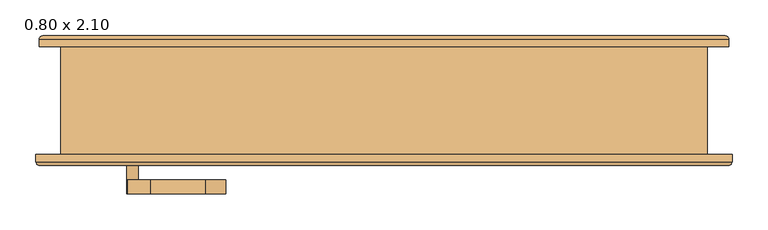
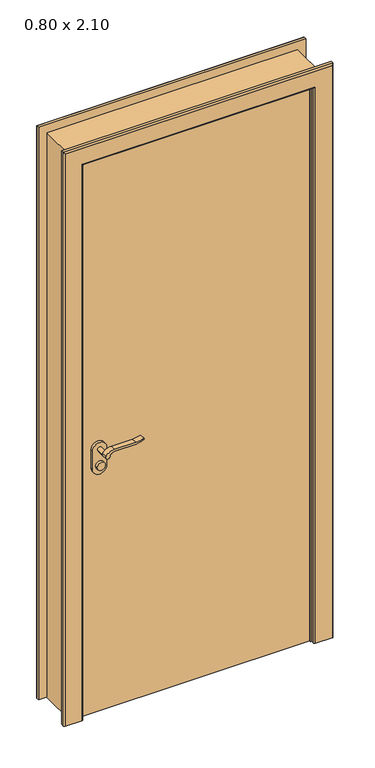
"""IFC4 building model written with IfcOpenShell, lengths in millimetres: door geometry, PORTA_DE_ABRIR_MADEIRA : 0.80 x 2.10."""

from ifc_helpers import new_model, si_unit, point, frame, frame_2d, origin, origin_with_axes, place, context, project, spatial, polyline, circle_curve, ellipse_curve, trimmed, segment, composite_curve, outline, extrude, faceted_brep, source, transform, mapped, element, save
from ifc_brep_helpers import plane_surface, cylinder_surface, advanced_brep


def door_0_80_x_2_10_69306b0e(model_context):
    return source(origin(), model_context, "Body", "SolidModel", [
        extrude(outline(composite_curve([segment(trimmed(circle_curve(frame_2d((940.0, -350.0)), 15.0), [point((940.0, -335.0))], [point((940.0, -365.0))], False, "CARTESIAN"), True, "CONTINUOUS"), segment(trimmed(circle_curve(frame_2d((940.0, -350.0)), 15.0), [point((940.0, -365.0))], [point((940.0, -335.0))], False, "CARTESIAN"), True, "CONTINUOUS")], self_intersect=False)), frame((0.0, -25.0, 0.0), z_axis=(0.0, 1.0, 0.0), x_axis=(0.0, 0.0, 1.0)), (0.0, 0.0, 1.0), 10.0),
        extrude(outline(composite_curve([segment(trimmed(circle_curve(frame_2d((940.0, -350.0)), 15.0), [point((940.0, -335.0))], [point((940.0, -365.0))], False, "CARTESIAN"), True, "CONTINUOUS"), segment(trimmed(circle_curve(frame_2d((940.0, -350.0)), 15.0), [point((940.0, -365.0))], [point((940.0, -335.0))], False, "CARTESIAN"), True, "CONTINUOUS")], self_intersect=False)), frame((0.0, -90.0, 0.0), z_axis=(0.0, 1.0, 0.0), x_axis=(0.0, 0.0, 1.0)), (0.0, 0.0, 1.0), 10.0),
        extrude(outline(composite_curve([segment(trimmed(circle_curve(frame_2d((1000.0, -350.0)), 8.0), [point((1004.6523287, -356.5081363))], [point((1000.0, -342.0))], False, "CARTESIAN"), True, "CONTINUOUS"), segment(trimmed(circle_curve(frame_2d((994.8738613, -324.6138099)), 18.1261387), [point((1000.0, -342.0))], [point((1013.0, -324.6138099))], True, "CARTESIAN"), True, "CONTINUOUS"), segment(polyline([(1013.0, -324.6138099), (1013.0, -248.3564091)]), True, "CONTINUOUS"), segment(trimmed(circle_curve(frame_2d((1072.2709207, -251.9396612)), 59.3791355), [point((1013.0, -248.3564091))], [point((1022.2135558, -220.0))], False, "CARTESIAN"), True, "CONTINUOUS"), segment(polyline([(1022.2135558, -220.0), (1025.0, -220.0)]), True, "CONTINUOUS"), segment(trimmed(circle_curve(frame_2d((1103.2850638, -248.4227909)), 83.2850902), [point((1025.0, -220.0))], [point((1020.0, -248.3564091))], True, "CARTESIAN"), True, "CONTINUOUS"), segment(polyline([(1020.0, -248.3564091), (1020.0, -324.6325667)]), True, "CONTINUOUS"), segment(trimmed(circle_curve(frame_2d((982.7555521, -326.3324871)), 37.2832219), [point((1020.0, -324.6325667))], [point((1004.6523287, -356.5081363))], False, "CARTESIAN"), True, "CONTINUOUS")], self_intersect=False)), frame((0.0, 5.0, 0.0), z_axis=(0.0, 1.0, 0.0), x_axis=(0.0, 0.0, 1.0)), (0.0, 0.0, 1.0), 20.0),
        extrude(outline(composite_curve([segment(trimmed(circle_curve(frame_2d((994.8738682, -324.6138122)), 18.1261318), [point((999.9999903, -342.0))], [point((1013.0, -324.6138122))], True, "CARTESIAN"), True, "CONTINUOUS"), segment(polyline([(1013.0, -324.6138122), (1013.0, -248.3564091)]), True, "CONTINUOUS"), segment(trimmed(circle_curve(frame_2d((1072.2709207, -251.9396612)), 59.3791355), [point((1013.0, -248.3564091))], [point((1022.2135558, -220.0))], False, "CARTESIAN"), True, "CONTINUOUS"), segment(polyline([(1022.2135558, -220.0), (1025.0, -220.0)]), True, "CONTINUOUS"), segment(trimmed(circle_curve(frame_2d((1103.2850638, -248.4227909)), 83.2850902), [point((1025.0, -220.0))], [point((1020.0, -248.3564091))], True, "CARTESIAN"), True, "CONTINUOUS"), segment(polyline([(1020.0, -248.3564091), (1020.0, -324.6325667)]), True, "CONTINUOUS"), segment(trimmed(circle_curve(frame_2d((982.7555521, -326.3324871)), 37.2832219), [point((1020.0, -324.6325667))], [point((1004.6523287, -356.5081363))], False, "CARTESIAN"), True, "CONTINUOUS"), segment(trimmed(circle_curve(frame_2d((1000.0, -350.0)), 8.0), [point((1004.6523287, -356.5081363))], [point((999.9999903, -342.0))], False, "CARTESIAN"), True, "CONTINUOUS")], self_intersect=False)), frame((0.0, -130.0, 0.0), z_axis=(0.0, 1.0, 0.0), x_axis=(0.0, 0.0, 1.0)), (0.0, 0.0, 1.0), 20.0),
        extrude(outline(composite_curve([segment(trimmed(circle_curve(frame_2d((1000.0, -350.0)), 8.0), [point((1000.0, -342.0))], [point((1000.0, -358.0))], False, "CARTESIAN"), True, "CONTINUOUS"), segment(trimmed(circle_curve(frame_2d((1000.0, -350.0)), 8.0), [point((1000.0, -358.0))], [point((1000.0, -342.0))], False, "CARTESIAN"), True, "CONTINUOUS")], self_intersect=False)), frame((0.0, -25.0, 0.0), z_axis=(0.0, 1.0, 0.0), x_axis=(0.0, 0.0, 1.0)), (0.0, 0.0, 1.0), 30.0),
        extrude(outline(composite_curve([segment(trimmed(circle_curve(frame_2d((1000.0, -350.0)), 8.0), [point((1000.0, -342.0))], [point((1000.0, -358.0))], False, "CARTESIAN"), True, "CONTINUOUS"), segment(trimmed(circle_curve(frame_2d((1000.0, -350.0)), 8.0), [point((1000.0, -358.0))], [point((1000.0, -342.0))], False, "CARTESIAN"), True, "CONTINUOUS")], self_intersect=False)), frame((0.0, -110.0, 0.0), z_axis=(0.0, 1.0, 0.0), x_axis=(0.0, 0.0, 1.0)), (0.0, 0.0, 1.0), 30.0),
        extrude(outline(composite_curve([segment(trimmed(circle_curve(frame_2d((930.0, -350.0)), 25.0), [point((930.0, -375.0))], [point((930.0, -325.0))], False, "CARTESIAN"), True, "CONTINUOUS"), segment(polyline([(930.0, -325.0), (1000.0, -325.0)]), True, "CONTINUOUS"), segment(trimmed(circle_curve(frame_2d((1000.0, -350.0)), 25.0), [point((1000.0, -325.0))], [point((1000.0, -375.0))], False, "CARTESIAN"), True, "CONTINUOUS"), segment(polyline([(1000.0, -375.0), (930.0, -375.0)]), True, "CONTINUOUS")], self_intersect=False)), frame((0.0, -35.0, 0.0), z_axis=(0.0, 1.0, 0.0), x_axis=(0.0, 0.0, 1.0)), (0.0, 0.0, 1.0), 10.0),
        extrude(outline(composite_curve([segment(trimmed(circle_curve(frame_2d((930.0, -350.0)), 25.0), [point((930.0, -375.0))], [point((930.0, -325.0))], False, "CARTESIAN"), True, "CONTINUOUS"), segment(polyline([(930.0, -325.0), (1000.0, -325.0)]), True, "CONTINUOUS"), segment(trimmed(circle_curve(frame_2d((1000.0, -350.0)), 25.0), [point((1000.0, -325.0))], [point((1000.0, -375.0))], False, "CARTESIAN"), True, "CONTINUOUS"), segment(polyline([(1000.0, -375.0), (930.0, -375.0)]), True, "CONTINUOUS")], self_intersect=False)), frame((0.0, -80.0, 0.0), z_axis=(0.0, 1.0, 0.0), x_axis=(0.0, 0.0, 1.0)), (0.0, 0.0, 1.0), 10.0),
        faceted_brep([(-410.0, -35.0, 0.0), (-410.0, -75.0, 0.0), (-450.0, -75.0, 0.0), (-450.0, 75.0, 0.0), (-400.0, 75.0, 0.0), (-400.0, -35.0, 0.0), (-410.0, -35.0, 2100.0), (-410.0, -75.0, 2100.0), (410.0, -75.0, 2100.0), (410.0, -75.0, 0.0), (450.0, -75.0, 0.0), (450.0, -75.0, 2140.0), (-450.0, -75.0, 2140.0), (-450.0, 75.0, 2140.0), (450.0, 75.0, 2140.0), (450.0, 75.0, 0.0), (400.0, 75.0, 0.0), (400.0, 75.0, 2090.0), (-400.0, 75.0, 2090.0), (-400.0, -35.0, 2090.0), (400.0, -35.0, 2090.0), (400.0, -35.0, 0.0), (410.0, -35.0, 0.0), (410.0, -35.0, 2100.0)], [[[0, 1, 2, 3, 4, 5]], [[1, 0, 6, 7]], [[2, 1, 7, 8, 9, 10, 11, 12]], [[3, 2, 12, 13]], [[4, 3, 13, 14, 15, 16, 17, 18]], [[5, 4, 18, 19]], [[0, 5, 19, 20, 21, 22, 23, 6]], [[20, 17, 16, 21]], [[22, 21, 16, 15, 10, 9]], [[8, 23, 22, 9]], [[14, 11, 10, 15]], [[13, 12, 11, 14]], [[19, 18, 17, 20]], [[7, 6, 23, 8]]]),
        advanced_brep(
        [(-480.0, 75.3, 0.0), (-480.0, 85.3, 0.0), (-475.0, 90.3, 0.0), (-415.0, 90.3, 0.0), (-410.0, 85.3, 0.0), (-410.0, 75.3, 0.0), (-480.0, 75.3, 2170.0), (-480.0, 85.3, 2170.0), (-475.0, 90.3, 2165.0), (475.0, 90.3, 2165.0), (475.0, 90.3, 0.0), (415.0, 90.3, 0.0), (415.0, 90.3, 2105.0), (-415.0, 90.3, 2105.0), (-410.0, 85.3, 2100.0), (-410.0, 75.3, 2100.0), (410.0, 75.3, 2100.0), (410.0, 75.3, 0.0), (480.0, 75.3, 0.0), (480.0, 75.3, 2170.0), (410.0, 85.3, 0.0), (480.0, 85.3, 0.0), (410.0, 85.3, 2100.0), (480.0, 85.3, 2170.0)],
        [
            (0, 1),
            (1, 2, circle_curve(frame((-475.0, 85.3, 0.0), z_axis=(0.0, 0.0, -1.0), x_axis=(-1.0, 0.0, 0.0)), 5.0)),
            (2, 3),
            (3, 4, circle_curve(frame((-415.0, 85.3, 0.0), z_axis=(0.0, 0.0, -1.0), x_axis=(-1.0, 0.0, 0.0)), 5.0)),
            (4, 5),
            (5, 0),
            (0, 6),
            (6, 7),
            (7, 1),
            (7, 8, ellipse_curve(frame((-475.0, 85.3, 2165.0), z_axis=(-0.7071067811865475, 0.0, -0.7071067811865475), x_axis=(0.7071067811865474, 0.0, -0.7071067811865476)), 7.0710678, 5.0)),
            (8, 2),
            (8, 9),
            (9, 10),
            (10, 11),
            (11, 12),
            (12, 13),
            (13, 3),
            (13, 14, ellipse_curve(frame((-415.0, 85.3, 2105.0), z_axis=(-0.7071067811865475, 0.0, -0.7071067811865475), x_axis=(0.7071067811865474, 0.0, -0.7071067811865476)), 7.0710678, 5.0)),
            (14, 4),
            (14, 15),
            (15, 5),
            (15, 16),
            (16, 17),
            (17, 18),
            (18, 19),
            (19, 6),
            (17, 20),
            (20, 11, circle_curve(frame((415.0, 85.3, 0.0), z_axis=(0.0, 0.0, -1.0), x_axis=(1.0, 0.0, 0.0)), 5.0)),
            (10, 21, circle_curve(frame((475.0, 85.3, 0.0), z_axis=(0.0, 0.0, -1.0), x_axis=(1.0, 0.0, 0.0)), 5.0)),
            (21, 18),
            (16, 22),
            (22, 20),
            (22, 12, ellipse_curve(frame((415.0, 85.3, 2105.0), z_axis=(0.7071067811865475, 0.0, -0.7071067811865475), x_axis=(0.7071067811865474, 0.0, 0.7071067811865476)), 7.0710678, 5.0)),
            (9, 23, ellipse_curve(frame((475.0, 85.3, 2165.0), z_axis=(0.7071067811865475, 0.0, -0.7071067811865475), x_axis=(0.7071067811865474, 0.0, 0.7071067811865476)), 7.0710678, 5.0)),
            (23, 21),
            (23, 19),
            (23, 7),
            (14, 22),
        ],
        [
            plane_surface(frame((-450.0, -75.0, 0.0), z_axis=(0.0, 0.0, -1.0), x_axis=(0.0, -1.0, 0.0))),
            plane_surface(frame((-480.0, 75.3, 0.0), z_axis=(-1.0, 0.0, 0.0), x_axis=(0.0, 0.0, 1.0))),
            cylinder_surface(frame((-475.0, 85.3, 0.0), z_axis=(0.0, 0.0, -1.0), x_axis=(-1.0, 0.0, 0.0)), 5.0),
            plane_surface(frame((-475.0, 90.3, 0.0), z_axis=(0.0, 1.0, 0.0), x_axis=(0.0, 0.0, 1.0))),
            cylinder_surface(frame((-415.0, 85.3, 0.0), z_axis=(0.0, 0.0, -1.0), x_axis=(-1.0, 0.0, 0.0)), 5.0),
            plane_surface(frame((-410.0, 85.3, 0.0), z_axis=(1.0, 0.0, 0.0), x_axis=(0.0, 0.0, 1.0))),
            plane_surface(frame((-410.0, 75.3, 0.0), z_axis=(0.0, -1.0, 0.0), x_axis=(0.0, 0.0, 1.0))),
            plane_surface(frame((450.0, -75.0, 0.0), z_axis=(0.0, 0.0, -1.0), x_axis=(0.0, -1.0, 0.0))),
            plane_surface(frame((410.0, 85.3, 2100.0), z_axis=(-1.0, 0.0, 0.0), x_axis=(0.0, 0.0, -1.0))),
            cylinder_surface(frame((415.0, 85.3, 2140.0), z_axis=(0.0, 0.0, 1.0), x_axis=(1.0, 0.0, 0.0)), 5.0),
            cylinder_surface(frame((475.0, 85.3, 2140.0), z_axis=(0.0, 0.0, 1.0), x_axis=(1.0, 0.0, 0.0)), 5.0),
            plane_surface(frame((480.0, 75.3, 2170.0), z_axis=(1.0, 0.0, 0.0), x_axis=(0.0, 0.0, -1.0))),
            plane_surface(frame((-480.0, 75.3, 2170.0), z_axis=(0.0, 0.0, 1.0), x_axis=(1.0, 0.0, 0.0))),
            plane_surface(frame((-410.0, 85.3, 2100.0), z_axis=(0.0, 0.0, -1.0), x_axis=(1.0, 0.0, 0.0))),
            cylinder_surface(frame((-450.0, 85.3, 2165.0), z_axis=(-1.0, 0.0, 0.0), x_axis=(0.0, 0.0, 1.0)), 5.0),
            cylinder_surface(frame((-450.0, 85.3, 2105.0), z_axis=(-1.0, 0.0, 0.0), x_axis=(0.0, 0.0, 1.0)), 5.0),
        ],
        [
            (0, [[1, 2, 3, 4, 5, 6]]),
            (1, [[-1, 7, 8, 9]]),
            (2, [[-2, -9, 10, 11]]),
            (3, [[-3, -11, 12, 13, 14, 15, 16, 17]]),
            (4, [[-4, -17, 18, 19]]),
            (5, [[-5, -19, 20, 21]]),
            (6, [[-6, -21, 22, 23, 24, 25, 26, -7]]),
            (7, [[-24, 27, 28, -14, 29, 30]]),
            (8, [[31, 32, -27, -23]]),
            (9, [[33, -15, -28, -32]]),
            (10, [[34, 35, -29, -13]]),
            (11, [[36, -25, -30, -35]]),
            (12, [[-8, -26, -36, 37]]),
            (13, [[-20, 38, -31, -22]]),
            (14, [[-10, -37, -34, -12]]),
            (15, [[-18, -16, -33, -38]]),
        ],
    ),
        advanced_brep(
        [(-479.3155593, -90.2647517, 0.0), (-484.3155593, -85.2647517, 0.0), (-484.3155593, -75.2647517, 0.0), (-414.3155593, -75.2647517, 0.0), (-414.3155593, -85.2647517, 0.0), (-419.3155593, -90.2647517, 0.0), (-479.3155593, -90.2647517, 2169.3155593), (-484.3155593, -85.2647517, 2174.3155593), (-484.3155593, -75.2647517, 2174.3155593), (484.3155593, -75.2647517, 2174.3155593), (484.3155593, -75.2647517, 0.0), (414.3155593, -75.2647517, 0.0), (414.3155593, -75.2647517, 2104.3155593), (-414.3155593, -75.2647517, 2104.3155593), (-414.3155593, -85.2647517, 2104.3155593), (-419.3155593, -90.2647517, 2109.3155593), (419.3155593, -90.2647517, 2109.3155593), (419.3155593, -90.2647517, 0.0), (479.3155593, -90.2647517, 0.0), (479.3155593, -90.2647517, 2169.3155593), (414.3155593, -85.2647517, 0.0), (484.3155593, -85.2647517, 0.0), (414.3155593, -85.2647517, 2104.3155593), (484.3155593, -85.2647517, 2174.3155593)],
        [
            (0, 1, circle_curve(frame((-479.3155593, -85.2647517, 0.0), z_axis=(0.0, 0.0, -1.0), x_axis=(-1.0, 0.0, 0.0)), 5.0)),
            (1, 2),
            (2, 3),
            (3, 4),
            (4, 5, circle_curve(frame((-419.3155593, -85.2647517, 0.0), z_axis=(0.0, 0.0, -1.0), x_axis=(-1.0, 0.0, 0.0)), 5.0)),
            (5, 0),
            (0, 6),
            (6, 7, ellipse_curve(frame((-479.3155593, -85.2647517, 2169.3155593), z_axis=(-0.7071067811865475, 0.0, -0.7071067811865475), x_axis=(0.7071067811865474, 0.0, -0.7071067811865476)), 7.0710678, 5.0)),
            (7, 1),
            (7, 8),
            (8, 2),
            (8, 9),
            (9, 10),
            (10, 11),
            (11, 12),
            (12, 13),
            (13, 3),
            (13, 14),
            (14, 4),
            (14, 15, ellipse_curve(frame((-419.3155593, -85.2647517, 2109.3155593), z_axis=(-0.7071067811865475, 0.0, -0.7071067811865475), x_axis=(0.7071067811865474, 0.0, -0.7071067811865476)), 7.0710678, 5.0)),
            (15, 5),
            (15, 16),
            (16, 17),
            (17, 18),
            (18, 19),
            (19, 6),
            (17, 20, circle_curve(frame((419.3155593, -85.2647517, 0.0), z_axis=(0.0, 0.0, -1.0), x_axis=(1.0, 0.0, 0.0)), 5.0)),
            (20, 11),
            (10, 21),
            (21, 18, circle_curve(frame((479.3155593, -85.2647517, 0.0), z_axis=(0.0, 0.0, -1.0), x_axis=(1.0, 0.0, 0.0)), 5.0)),
            (16, 22, ellipse_curve(frame((419.3155593, -85.2647517, 2109.3155593), z_axis=(0.7071067811865475, 0.0, -0.7071067811865475), x_axis=(0.7071067811865474, 0.0, 0.7071067811865476)), 7.0710678, 5.0)),
            (22, 20),
            (22, 12),
            (9, 23),
            (23, 21),
            (23, 19, ellipse_curve(frame((479.3155593, -85.2647517, 2169.3155593), z_axis=(0.7071067811865475, 0.0, -0.7071067811865475), x_axis=(0.7071067811865474, 0.0, 0.7071067811865476)), 7.0710678, 5.0)),
            (7, 23),
            (22, 14),
        ],
        [
            plane_surface(frame((-450.0, -75.0, 0.0), z_axis=(0.0, 0.0, -1.0), x_axis=(0.0, -1.0, 0.0))),
            cylinder_surface(frame((-479.3155593, -85.2647517, 0.0), z_axis=(0.0, 0.0, -1.0), x_axis=(-1.0, 0.0, 0.0)), 5.0),
            plane_surface(frame((-484.3155593, -85.2647517, 0.0), z_axis=(-1.0, 0.0, 0.0), x_axis=(0.0, 0.0, 1.0))),
            plane_surface(frame((-484.3155593, -75.2647517, 0.0), z_axis=(0.0, 1.0, 0.0), x_axis=(0.0, 0.0, 1.0))),
            plane_surface(frame((-414.3155593, -75.2647517, 0.0), z_axis=(1.0, 0.0, 0.0), x_axis=(0.0, 0.0, 1.0))),
            cylinder_surface(frame((-419.3155593, -85.2647517, 0.0), z_axis=(0.0, 0.0, -1.0), x_axis=(-1.0, 0.0, 0.0)), 5.0),
            plane_surface(frame((-419.3155593, -90.2647517, 0.0), z_axis=(0.0, -1.0, 0.0), x_axis=(0.0, 0.0, 1.0))),
            plane_surface(frame((450.0, -75.0, 0.0), z_axis=(0.0, 0.0, -1.0), x_axis=(0.0, -1.0, 0.0))),
            cylinder_surface(frame((419.3155593, -85.2647517, 2140.0), z_axis=(0.0, 0.0, 1.0), x_axis=(1.0, 0.0, 0.0)), 5.0),
            plane_surface(frame((414.3155593, -75.2647517, 2104.3155593), z_axis=(-1.0, 0.0, 0.0), x_axis=(0.0, 0.0, -1.0))),
            plane_surface(frame((484.3155593, -85.2647517, 2174.3155593), z_axis=(1.0, 0.0, 0.0), x_axis=(0.0, 0.0, -1.0))),
            cylinder_surface(frame((479.3155593, -85.2647517, 2140.0), z_axis=(0.0, 0.0, 1.0), x_axis=(1.0, 0.0, 0.0)), 5.0),
            plane_surface(frame((-484.3155593, -85.2647517, 2174.3155593), z_axis=(0.0, 0.0, 1.0), x_axis=(1.0, 0.0, 0.0))),
            plane_surface(frame((-414.3155593, -75.2647517, 2104.3155593), z_axis=(0.0, 0.0, -1.0), x_axis=(1.0, 0.0, 0.0))),
            cylinder_surface(frame((-450.0, -85.2647517, 2169.3155593), z_axis=(-1.0, 0.0, 0.0), x_axis=(0.0, 0.0, 1.0)), 5.0),
            cylinder_surface(frame((-450.0, -85.2647517, 2109.3155593), z_axis=(-1.0, 0.0, 0.0), x_axis=(0.0, 0.0, 1.0)), 5.0),
        ],
        [
            (0, [[1, 2, 3, 4, 5, 6]]),
            (1, [[-1, 7, 8, 9]]),
            (2, [[-2, -9, 10, 11]]),
            (3, [[-3, -11, 12, 13, 14, 15, 16, 17]]),
            (4, [[-4, -17, 18, 19]]),
            (5, [[-5, -19, 20, 21]]),
            (6, [[-6, -21, 22, 23, 24, 25, 26, -7]]),
            (7, [[-24, 27, 28, -14, 29, 30]]),
            (8, [[31, 32, -27, -23]]),
            (9, [[33, -15, -28, -32]]),
            (10, [[34, 35, -29, -13]]),
            (11, [[36, -25, -30, -35]]),
            (12, [[-10, 37, -34, -12]]),
            (13, [[-18, -16, -33, 38]]),
            (14, [[-8, -26, -36, -37]]),
            (15, [[-20, -38, -31, -22]]),
        ],
    ),
        extrude(outline(polyline([(410.0, -70.0), (-410.0, -70.0), (-410.0, -35.0), (410.0, -35.0), (410.0, -70.0)])), origin_with_axes(), (0.0, 0.0, 1.0), 2100.0),
    ])


if __name__ == "__main__":
    model = new_model("IFC4")
    model_context = context("Model", 3, world=origin())
    ifc_project = project(units=[si_unit("LENGTHUNIT", "METRE", prefix="MILLI")], contexts=[model_context])
    site = spatial("IfcSite", under=ifc_project)
    building = spatial("IfcBuilding", under=site)
    placement = place(None, origin())
    door_0_80_x_2_10_shape = door_0_80_x_2_10_69306b0e(model_context)
    element("IfcDoor", 1, ObjectType="PORTA_DE_ABRIR_MADEIRA : 0.80 x 2.10", at=placement, inside=building, context=model_context, shape_type="MappedRepresentation", body=[
        mapped(door_0_80_x_2_10_shape, transform((0.0, 0.0, 0.0), x_axis=(1.0, 0.0, 0.0), y_axis=(0.0, 1.0, 0.0), z_axis=(0.0, 0.0, 1.0))),
    ])
    save(model, "model.ifc")

# Revit data of these elements
# Type "PORTA_DE_ABRIR_MADEIRA : 0.80 x 2.10"
#   Type Mark = "P2"
#   Analytic Construction = "<Nenhum>"
#   Rough Width = 0.90 m
#   Projeção da estrutura externa = 0.50 m
#   Projeção da estrutura interna = 0.025 m
#   Largura da estrutura = 0.075 m
#   Rough Height = 2.15 m
#   Height = 2.10 m
#   Width = 0.80 m
#   Soleira [instance default] = no
#   Material do batente = .BATENTE E GUARNIÇÃO
#   Material da maçaneta = .AÇO INOXIDÁVEL ESCOVADO
#   Material da folha da porta = .FOLHA DA PORTA
#   Material da Soleira [instance default] = none
#   Function = (empty or 0)
#   Wall Closure = (empty or 0)
# Element 1 (IfcDoor, "PORTA_DE_ABRIR_MADEIRA : 0.80 x 2.10")
#   Materials on its faces: ".AÇO INOXIDÁVEL ESCOVADO", ".BATENTE E GUARNIÇÃO", ".FOLHA DA PORTA"
# Materials
#   ".BATENTE E GUARNIÇÃO": class "Madeira", colour RGB 215 186 156, transparency 0, Cost = 0
#   ".AÇO INOXIDÁVEL ESCOVADO": class "Metal", colour RGB 189 187 185, transparency 0, Description = "Stainless Steel 18/8, brushed finish", Cost = 0
#   ".FOLHA DA PORTA": class "Madeira", colour RGB 148 119 91, transparency 0, Cost = 0
